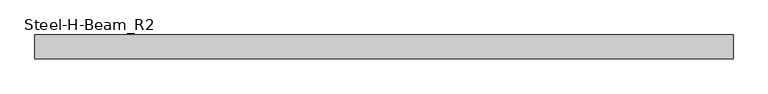
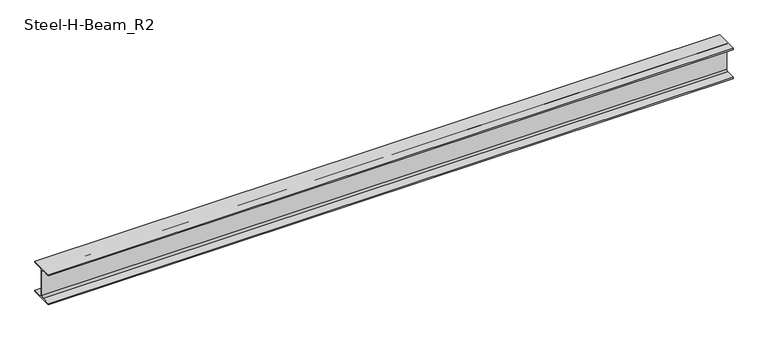
"""IFC4 building model written with IfcOpenShell, lengths in millimetres: beam geometry, Steel-H-Beam_R2 : BM121_H-340×250x9x14_SG1."""

import ifcopenshell
import ifcopenshell.guid

model = None  # the IFC model being written
_history = None  # IfcOwnerHistory: only IFC2X3 demands one
_inside = {}  # id of a spatial element -> (the spatial element, [elements in it])
_under = {}  # id of a project, library or spatial element -> (it, [spatial elements below it])
_declared = {}  # id of a project -> (the project, [libraries it declares])
_typed = {}  # id of a type object -> (the type object, [elements of that type])
_made_of = {}  # id of a material, layer set ... -> (it, [elements and type objects made of it])


def new_model(schema):
    """Start an empty IFC model of exactly this schema.

    Asked for "IFC4X3", IfcOpenShell would pick the latest addendum, in which some entities
    have other attributes; the version numbers below select the first issue.
    IFC2X3 requires an IfcOwnerHistory on every rooted entity: one is made here for all.
    """
    global model, _history
    if schema == "IFC4X3":
        model = ifcopenshell.file(schema_version=(4, 3, 0, 0))
    else:
        model = ifcopenshell.file(schema=schema)
    _inside.clear()
    _under.clear()
    _declared.clear()
    _typed.clear()
    _made_of.clear()
    _history = None
    if model.schema == "IFC2X3":
        org = make("IfcOrganization", Name="unknown")
        user = make(
            "IfcPersonAndOrganization",
            ThePerson=make("IfcPerson", FamilyName="unknown"),
            TheOrganization=org,
        )
        app = make(
            "IfcApplication",
            ApplicationDeveloper=org,
            Version="unknown",
            ApplicationFullName="unknown",
            ApplicationIdentifier="unknown",
        )
        _history = make(
            "IfcOwnerHistory",
            OwningUser=user,
            OwningApplication=app,
            ChangeAction="ADDED",
            CreationDate=0,
        )
    return model


def make(cls, **values):
    """One entity of the class cls with the attributes given. An attribute that is None is left unset."""
    return model.create_entity(
        cls, **{name: value for name, value in values.items() if value is not None}
    )


def rooted(cls, **values):
    """An entity with a GlobalId (a new one), such as an element, a storey or a relation."""
    return make(cls, GlobalId=ifcopenshell.guid.new(), OwnerHistory=_history, **values)


def si_unit(unit_type, name, prefix=None):
    """IfcSIUnit, for example si_unit("LENGTHUNIT", "METRE", prefix="MILLI")."""
    return make("IfcSIUnit", UnitType=unit_type, Prefix=prefix, Name=name)


def assignment(units):
    """IfcUnitAssignment: the units of a project."""
    return None if units is None else make("IfcUnitAssignment", Units=units)


def point(xyz):
    """IfcCartesianPoint."""
    return None if xyz is None else make("IfcCartesianPoint", Coordinates=xyz)


def direction(xyz):
    """IfcDirection."""
    return None if xyz is None else make("IfcDirection", DirectionRatios=xyz)


def frame(location, z_axis=None, x_axis=None):
    """IfcAxis2Placement3D, a coordinate frame: its origin and axes. An axis left out is left unset."""
    return make(
        "IfcAxis2Placement3D",
        Location=point(location),
        Axis=direction(z_axis),
        RefDirection=direction(x_axis),
    )


def frame_2d(location, x_axis=None):
    """IfcAxis2Placement2D, a coordinate frame in the plane: its origin and x axis."""
    return make(
        "IfcAxis2Placement2D", Location=point(location), RefDirection=direction(x_axis)
    )


def origin():
    """The frame at (0, 0, 0) with its axes left unset."""
    return frame((0.0, 0.0, 0.0))


def place(relative_to, where):
    """IfcLocalPlacement: puts the frame where relative to a parent placement (None: the world)."""
    return make(
        "IfcLocalPlacement", PlacementRelTo=relative_to, RelativePlacement=where
    )


def context(
    kind, dimensions, precision=None, world=None, true_north=None, identifier=None
):
    """IfcGeometricRepresentationContext, for example the 3D "Model" context."""
    return make(
        "IfcGeometricRepresentationContext",
        ContextIdentifier=identifier,
        ContextType=kind,
        CoordinateSpaceDimension=dimensions,
        Precision=precision,
        WorldCoordinateSystem=world,
        TrueNorth=true_north,
    )


def project(units=None, contexts=None):
    """IfcProject with its units and contexts."""
    return rooted(
        "IfcProject",
        Name="project",
        RepresentationContexts=contexts,
        UnitsInContext=assignment(units),
    )


def spatial(cls, under=None, at=None, **own):
    """A site, building, storey or space (cls), placed at a placement, below another one or the project."""
    s = rooted(cls, ObjectPlacement=at, **own)
    if under is not None:
        _under.setdefault(under.id(), (under, []))[1].append(s)
    return s


def polyline(points):
    """IfcPolyline through the points."""
    return make("IfcPolyline", Points=[point(p) for p in points])


def circle_curve(where, radius):
    """IfcCircle in the frame where."""
    return make("IfcCircle", Position=where, Radius=radius)


def trimmed(basis, trim1, trim2, sense, master):
    """IfcTrimmedCurve: the piece of a basis curve between two trims."""
    return make(
        "IfcTrimmedCurve",
        BasisCurve=basis,
        Trim1=trim1,
        Trim2=trim2,
        SenseAgreement=sense,
        MasterRepresentation=master,
    )


def segment(curve, same_sense, transition):
    """IfcCompositeCurveSegment."""
    return make(
        "IfcCompositeCurveSegment",
        Transition=transition,
        SameSense=same_sense,
        ParentCurve=curve,
    )


def composite_curve(segments, self_intersect=None):
    """IfcCompositeCurve: segments joined end to end."""
    return make("IfcCompositeCurve", Segments=segments, SelfIntersect=self_intersect)


def outline(outer, holes=None, kind="AREA"):
    """IfcArbitraryClosedProfileDef: a profile drawn as a closed curve; with holes, ...WithVoids."""
    if holes is None:
        return make("IfcArbitraryClosedProfileDef", ProfileType=kind, OuterCurve=outer)
    return make(
        "IfcArbitraryProfileDefWithVoids",
        ProfileType=kind,
        OuterCurve=outer,
        InnerCurves=holes,
    )


def extrude(swept, where, along, depth):
    """IfcExtrudedAreaSolid: the profile swept, set in the frame where, extruded along a direction by depth."""
    return make(
        "IfcExtrudedAreaSolid",
        SweptArea=swept,
        Position=where,
        ExtrudedDirection=direction(along),
        Depth=depth,
    )


def shape(context_of_items, identifier, shape_type, items):
    """IfcShapeRepresentation: the items that make up one representation, for example the "Body"."""
    return make(
        "IfcShapeRepresentation",
        ContextOfItems=context_of_items,
        RepresentationIdentifier=identifier,
        RepresentationType=shape_type,
        Items=items,
    )


def source(mapping_origin, context_of_items, identifier, shape_type, items):
    """IfcRepresentationMap: a shape defined once, which mapped items show again and again."""
    return make(
        "IfcRepresentationMap",
        MappingOrigin=mapping_origin,
        MappedRepresentation=shape(context_of_items, identifier, shape_type, items),
    )


def transform(
    local_origin,
    x_axis=None,
    y_axis=None,
    z_axis=None,
    scale=None,
    scale2=None,
    scale3=None,
    uniform=True,
):
    """IfcCartesianTransformationOperator3D, or its non-uniform kind. x_axis, y_axis, z_axis: its Axis1, 2, 3."""
    if uniform:
        return make(
            "IfcCartesianTransformationOperator3D",
            Axis1=direction(x_axis),
            Axis2=direction(y_axis),
            LocalOrigin=point(local_origin),
            Scale=scale,
            Axis3=direction(z_axis),
        )
    return make(
        "IfcCartesianTransformationOperator3DnonUniform",
        Axis1=direction(x_axis),
        Axis2=direction(y_axis),
        LocalOrigin=point(local_origin),
        Scale=scale,
        Axis3=direction(z_axis),
        Scale2=scale2,
        Scale3=scale3,
    )


def mapped(mapping_source, mapping_target):
    """IfcMappedItem: shows the shape of a source again, moved by a transform."""
    return make(
        "IfcMappedItem", MappingSource=mapping_source, MappingTarget=mapping_target
    )


def made_of(thing, what):
    """Note that an element or type object is made of a material, layer set ...; save() writes the relation."""
    if what is not None:
        _made_of.setdefault(what.id(), (what, []))[1].append(thing)
    return thing


def element(
    cls,
    number,
    at=None,
    inside=None,
    cuts=None,
    type_object=None,
    material=None,
    context=None,
    identifier="Body",
    shape_type=None,
    held_by="IfcProductDefinitionShape",
    body=None,
    shapes=None,
    **own,
):
    """One element of the class cls, such as IfcWall. Its Tag is "e" and its number.

    at: its placement. inside: the storey or other place that contains it. cuts: it is an
    opening in that element (IfcRelVoidsElement). A single representation is given by context,
    identifier, shape_type and body (its items); several are given by shapes. held_by: the class
    of the entity that holds the representations. save() writes the other relations.
    """
    e = rooted(cls, Tag="e%d" % number, ObjectPlacement=at, **own)
    if body is not None:
        shapes = [shape(context, identifier, shape_type, body)]
    if shapes is not None:
        e.Representation = make(held_by, Representations=shapes)
    if inside is not None:
        _inside.setdefault(inside.id(), (inside, []))[1].append(e)
    if cuts is not None:
        rooted(
            "IfcRelVoidsElement", RelatingBuildingElement=cuts, RelatedOpeningElement=e
        )
    if type_object is not None:
        _typed.setdefault(type_object.id(), (type_object, []))[1].append(e)
    return made_of(e, material)


def aggregate(whole, parts):
    """IfcRelAggregates: a whole, such as a stair, and the parts it consists of."""
    return rooted("IfcRelAggregates", RelatingObject=whole, RelatedObjects=parts)


def save(model, path):
    """Write the relations noted so far, then the file.

    IfcRelAggregates (storeys below a building ...), IfcRelContainedInSpatialStructure (elements
    in a storey), IfcRelDefinesByType, IfcRelAssociatesMaterial and IfcRelDeclares: one each for
    every whole, place, type object, material and project.
    """
    for whole, parts in _under.values():
        aggregate(whole, parts)
    for where, things in _inside.values():
        rooted(
            "IfcRelContainedInSpatialStructure",
            RelatedElements=things,
            RelatingStructure=where,
        )
    for kind, things in _typed.values():
        rooted("IfcRelDefinesByType", RelatedObjects=things, RelatingType=kind)
    for what, things in _made_of.values():
        rooted("IfcRelAssociatesMaterial", RelatedObjects=things, RelatingMaterial=what)
    for by, libraries in _declared.values():
        rooted("IfcRelDeclares", RelatingContext=by, RelatedDefinitions=libraries)
    model.write(path)


def steel_h_beam_r2_7d9a1970(model_context):
    return source(origin(), model_context, "Body", "SweptSolid", [
        extrude(outline(composite_curve([segment(polyline([(125.0, -156.0), (125.0, -170.0), (-125.0, -170.0), (-125.0, -156.0), (-24.5, -156.0)]), True, "CONTINUOUS"), segment(trimmed(circle_curve(frame_2d((-24.5, -136.0)), 20.0), [point((-24.5, -156.0))], [point((-4.5, -136.0))], True, "CARTESIAN"), True, "CONTINUOUS"), segment(polyline([(-4.5, -136.0), (-4.5, 136.0)]), True, "CONTINUOUS"), segment(trimmed(circle_curve(frame_2d((-24.5, 136.0)), 20.0), [point((-4.5, 136.0))], [point((-24.5, 156.0))], True, "CARTESIAN"), True, "CONTINUOUS"), segment(polyline([(-24.5, 156.0), (-125.0, 156.0), (-125.0, 170.0), (125.0, 170.0), (125.0, 156.0), (24.5, 156.0)]), True, "CONTINUOUS"), segment(trimmed(circle_curve(frame_2d((24.5, 136.0)), 20.0), [point((24.5, 156.0))], [point((4.5, 136.0))], True, "CARTESIAN"), True, "CONTINUOUS"), segment(polyline([(4.5, 136.0), (4.5, -136.0)]), True, "CONTINUOUS"), segment(trimmed(circle_curve(frame_2d((24.5, -136.0)), 20.0), [point((4.5, -136.0))], [point((24.5, -156.0))], True, "CARTESIAN"), True, "CONTINUOUS"), segment(polyline([(24.5, -156.0), (125.0, -156.0)]), True, "CONTINUOUS")], self_intersect=False)), frame((-4287.3, 0.0, 0.0), z_axis=(1.0, 0.0, 0.0), x_axis=(0.0, 1.0, 0.0)), (0.0, 0.0, 1.0), 7287.3),
    ])


if __name__ == "__main__":
    model = new_model("IFC4")
    model_context = context("Model", 3, world=origin())
    ifc_project = project(units=[si_unit("LENGTHUNIT", "METRE", prefix="MILLI")], contexts=[model_context])
    site = spatial("IfcSite", under=ifc_project)
    building = spatial("IfcBuilding", under=site)
    placement = place(None, origin())
    steel_h_beam_r2_shape = steel_h_beam_r2_7d9a1970(model_context)
    element("IfcBeam", 1, ObjectType="Steel-H-Beam_R2 : BM121_H-340×250x9x14_SG1", at=placement, inside=building, context=model_context, shape_type="MappedRepresentation", body=[
        mapped(steel_h_beam_r2_shape, transform((0.0, 0.0, 0.0), x_axis=(1.0, 0.0, 0.0), y_axis=(0.0, 1.0, 0.0), z_axis=(0.0, 0.0, 1.0))),
    ])
    save(model, "model.ifc")

# Revit data of these elements
# Type "Steel-H-Beam_R2 : BM121_H-340×250x9x14_SG1"
#   SteelWeight = "Medium"
#   Surface Area = 1.62766 m²/m
#   Section Area = 101.514 cm²
#   Mass per Unit Length = 79.6882 kg/m
#   Length [instance default] = 3000 mm
#   B = 250 mm
#   H = 340 mm
#   r = 20 mm
#   tw = 9 mm
#   tf = 14 mm
#   hec_material4 [instance default] = none
#   hec_material3 [instance default] = none
#   hec_material2 [instance default] = none
#   hec_material1 [instance default] = none
#   Structural Material [instance default] = Steel, 45-345
#   Assembly Code = ""
# Element 1 (IfcBeam, "Steel-H-Beam_R2 : BM121_H-340×250x9x14_SG1")
#   Materials on its faces: "Steel, 45-345"
# Materials
#   "Steel, 45-345": class "Metal", colour RGB 189 187 185, transparency 0, Description = "Steel 345 MPa", Cost = 0
